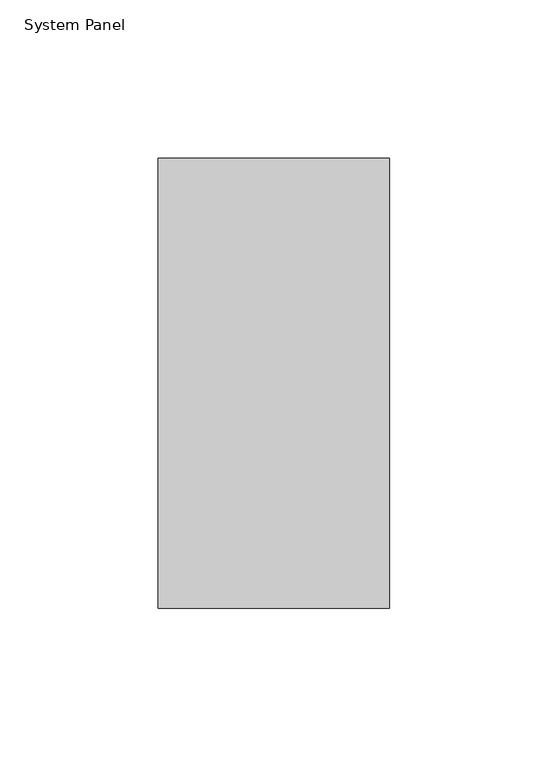
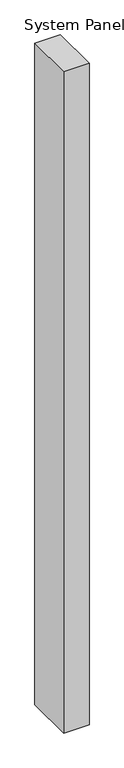
"""IFC4 building model written with IfcOpenShell, lengths in millimetres: plate geometry, System Panel : NLRS_21_CWP_hsb-vulling minerale wol 142 _gen_rsf."""

from ifc_helpers import new_model, si_unit, origin, origin_with_axes, place, context, project, spatial, polyline, outline, extrude, source, transform, mapped, element, save


def system_panel_19d5cf6b(model_context):
    return source(origin(), model_context, "Body", "SweptSolid", [
        extrude(outline(polyline([(36.5, -71.0), (-36.5, -71.0), (-36.5, 71.0), (36.5, 71.0), (36.5, -71.0)])), origin_with_axes(), (0.0, 0.0, 1.0), 2000.0),
    ])


if __name__ == "__main__":
    model = new_model("IFC4")
    model_context = context("Model", 3, world=origin())
    ifc_project = project(units=[si_unit("LENGTHUNIT", "METRE", prefix="MILLI")], contexts=[model_context])
    site = spatial("IfcSite", under=ifc_project)
    building = spatial("IfcBuilding", under=site)
    placement = place(None, origin())
    system_panel_shape = system_panel_19d5cf6b(model_context)
    element("IfcPlate", 1, ObjectType="System Panel : NLRS_21_CWP_hsb-vulling minerale wol 142 _gen_rsf", at=placement, inside=building, context=model_context, shape_type="MappedRepresentation", body=[
        mapped(system_panel_shape, transform((0.0, 0.0, 0.0), x_axis=(1.0, 0.0, 0.0), y_axis=(0.0, 1.0, 0.0), z_axis=(0.0, 0.0, 1.0))),
    ])
    save(model, "model.ifc")

# Revit data of these elements
# Type "System Panel : NLRS_21_CWP_hsb-vulling minerale wol 142 _gen_rsf"
#   Export Type to IFC As = "IfcWall"
#   Type IfcGUID = "07M7mRoiH1CR8m_RSKIwpC"
#   Assembly Code = "21.23"
# Element 1 (IfcPlate, "System Panel : NLRS_21_CWP_hsb-vulling minerale wol 142 _gen_rsf")
#   Materials on its faces: "NLRS_m1_isolatie minerale wol_gen_rsf"
# Materials
#   "NLRS_m1_isolatie minerale wol_gen_rsf": class "M - Anorganische materialen", colour RGB 200 200 140, transparency 0, Keynote = "m1", Manufacturer = "Revit Standards Foundation", URL = "www.revitstandards.org", Description = "isolatie minerale wol", Cost = 0
